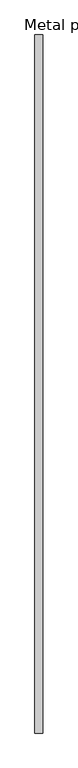
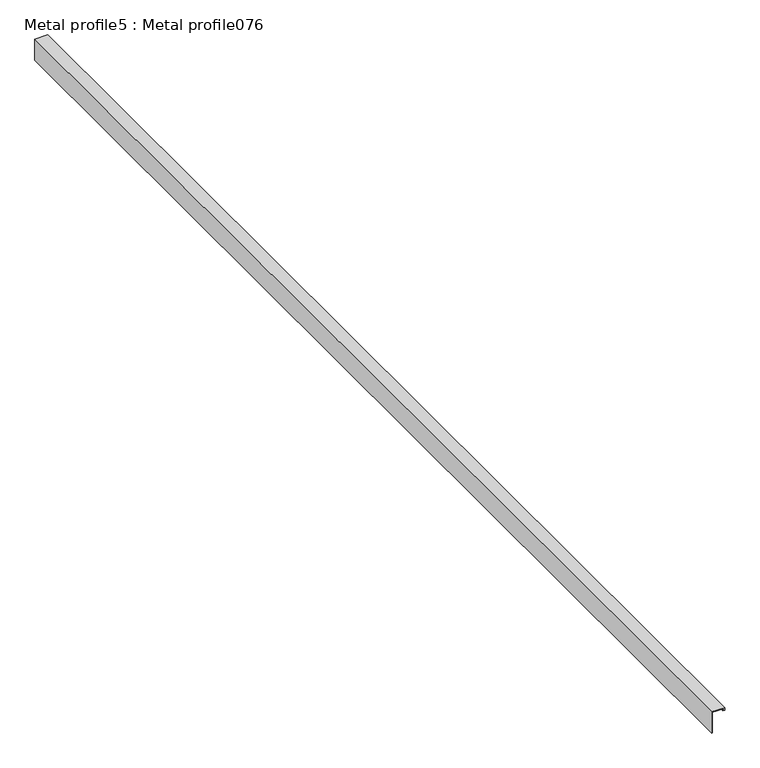
"""IFC4 building model written with IfcOpenShell, lengths in millimetres: proxy geometry, Metal profile5 : Metal profile076."""

from ifc_helpers import new_model, si_unit, frame, origin, place, context, project, spatial, polyline, outline, extrude, source, transform, mapped, element, save


def metal_profile5_metal_profile076_f0a74c49(model_context):
    return source(origin(), model_context, "Body", "SweptSolid", [
        extrude(outline(polyline([(40120.4288738, -9287.2762348), (40120.4288738, -9267.5912348), (40118.2190738, -9267.5912348), (40118.2190738, -9269.3236911), (40116.9490738, -9269.3236911), (40116.9490738, -9266.3212348), (40121.6988738, -9266.3212348), (40121.6988738, -9288.5462348), (40083.5988738, -9288.5462348), (40083.5988738, -9287.2762348), (40120.4288738, -9287.2762348)])), frame((0.0, 7182.1531721, 0.0), z_axis=(0.0, 1.0, 0.0), x_axis=(0.0, 0.0, 1.0)), (0.0, 0.0, 1.0), 2000.0),
    ])


if __name__ == "__main__":
    model = new_model("IFC4")
    model_context = context("Model", 3, world=origin())
    ifc_project = project(units=[si_unit("LENGTHUNIT", "METRE", prefix="MILLI")], contexts=[model_context])
    site = spatial("IfcSite", under=ifc_project)
    building = spatial("IfcBuilding", under=site)
    placement = place(None, origin())
    metal_profile5_metal_profile076_shape = metal_profile5_metal_profile076_f0a74c49(model_context)
    element("IfcBuildingElementProxy", 1, Name="Metal profile5 : Metal profile076", ObjectType="Metal profile5 : Metal profile076", at=placement, inside=building, context=model_context, shape_type="MappedRepresentation", body=[
        mapped(metal_profile5_metal_profile076_shape, transform((0.0, 0.0, 0.0), x_axis=(1.0, 0.0, 0.0), y_axis=(0.0, 1.0, 0.0), z_axis=(0.0, 0.0, 1.0))),
    ])
    save(model, "model.ifc")

# Revit data of these elements
# Type "Metal profile5 : Metal profile076"
#   NameOverride = "Metal profile076"
# Element 1 (IfcBuildingElementProxy, "Metal profile5 : Metal profile076")
#   Materials on its faces: "COPPER STUCCO J BEAD"
# Materials
#   "COPPER STUCCO J BEAD": class "Unassigned", colour RGB 251 232 155, transparency 0, Cost = 0
